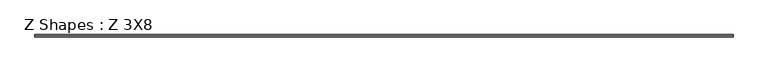
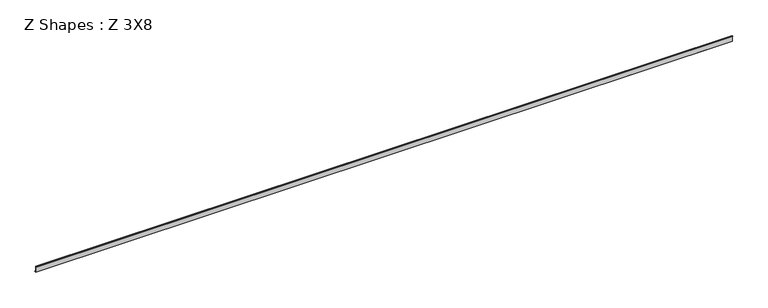
"""IFC4 building model written with IfcOpenShell, lengths in millimetres: beam geometry, Z Shapes : Z 3X8."""

from ifc_helpers import new_model, si_unit, frame, origin, place, context, project, spatial, polyline, outline, extrude, source, transform, mapped, element, save


def z_shapes_z_3x8_2a0398e4(model_context):
    return source(origin(), model_context, "Body", "SweptSolid", [
        extrude(outline(polyline([(-57.2805719, 92.452825), (-57.2805719, 102.104825), (-19.1805719, 102.104825), (-19.1805719, -92.459175), (18.9194281, -92.459175), (18.9194281, -98.809175), (-27.1991352, -98.809175), (-27.1991352, 92.452825), (-57.2805719, 92.452825)])), frame((-11474.45, 0.0, 0.0), z_axis=(1.0, 0.0, 0.0), x_axis=(0.0, 1.0, 0.0)), (0.0, 0.0, 1.0), 23361.65),
    ])


if __name__ == "__main__":
    model = new_model("IFC4")
    model_context = context("Model", 3, world=origin())
    ifc_project = project(units=[si_unit("LENGTHUNIT", "METRE", prefix="MILLI")], contexts=[model_context])
    site = spatial("IfcSite", under=ifc_project)
    building = spatial("IfcBuilding", under=site)
    placement = place(None, origin())
    z_shapes_z_3x8_shape = z_shapes_z_3x8_2a0398e4(model_context)
    element("IfcBeam", 1, ObjectType="Z Shapes : Z 3X8", at=placement, inside=building, context=model_context, shape_type="MappedRepresentation", body=[
        mapped(z_shapes_z_3x8_shape, transform((0.0, 0.0, 0.0), x_axis=(1.0, 0.0, 0.0), y_axis=(0.0, 1.0, 0.0), z_axis=(0.0, 0.0, 1.0))),
    ])
    save(model, "model.ifc")

# Revit data of these elements
# Type "Z Shapes : Z 3X8"
#   Section Name Key = "W12x26"
#   Assembly Code = "B10"
#   Width = 76.2 mm
#   Web Thickness = 5.842 mm
#   Web Fillet = 7.62 mm
#   Warping Constant = 163001.3 cm⁶
#   Torsional Moment of Inertia = 12.4869 cm⁴
#   Section Area = 7.65 in²
#   Plastic Modulus weak axis = 0.00472801 (stored number, unit not read)
#   Plastic Modulus strong axis = 0.0215278 (stored number, unit not read)
#   Perimeter = 15.0571 m²/m
#   Nominal Weight = 379.441 N/m
#   Moment of Inertia weak axis = 720.08 cm⁴
#   Moment of Inertia strong axis = 8491.12 cm⁴
#   Height = 184.912 mm
#   Flange Thickness = 9.652 mm
#   Elastic Modulus weak axis = 0.00309028 (stored number, unit not read)
#   Elastic Modulus strong axis = 0.0193287 (stored number, unit not read)
#   Centroid Vertical = 92.456 mm
#   Centroid Horizontal = 38.1 mm
#   Length [instance default] = 5' - 0"
#   Structural Material [instance default] = Steel ASTM A992
#   Principal Axes Angle = 0
# Element 1 (IfcBeam, "Z Shapes : Z 3X8")
#   Materials on its faces: "Steel ASTM A992"
# Materials
#   "Steel ASTM A992": class "Metal", colour RGB 189 187 185, transparency 0, Description = "Structural steel 50ksi", Cost = 0
